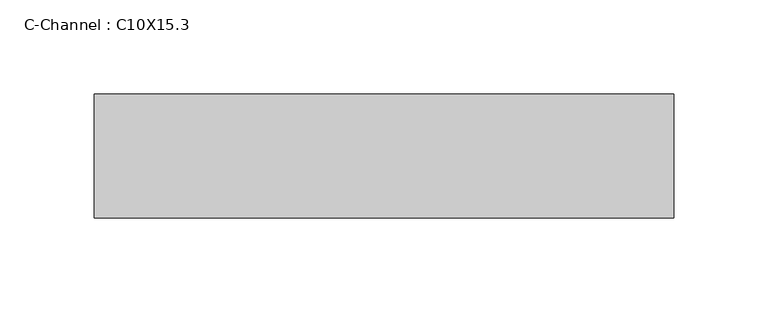
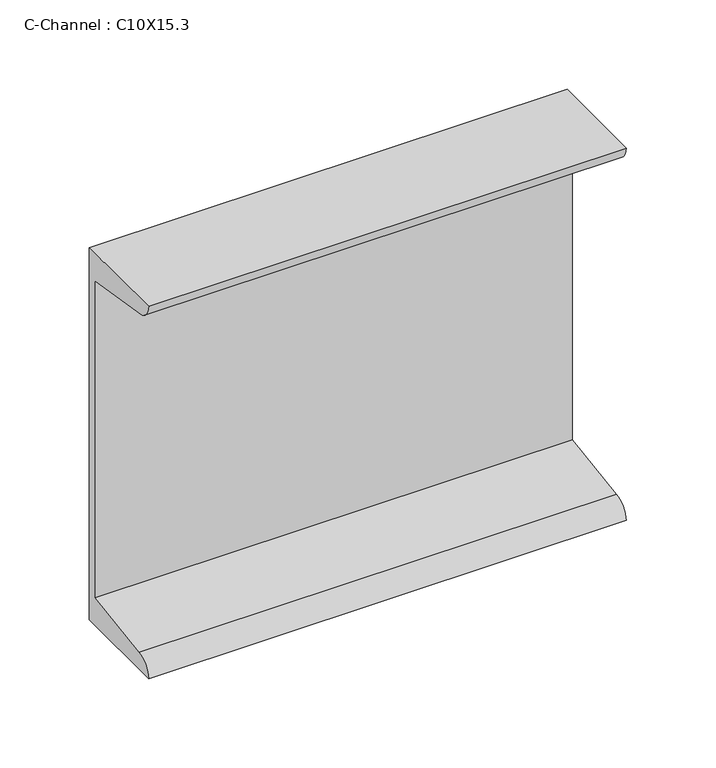
"""IFC4 building model written with IfcOpenShell, lengths in millimetres: beam geometry, C-Channel : C10X15.3."""

from ifc_helpers import new_model, si_unit, point, frame, frame_2d, origin, place, context, project, spatial, polyline, circle_curve, trimmed, segment, composite_curve, outline, extrude, source, transform, mapped, element, save


def c_channel_c10x15_3_af99d691(model_context):
    return source(origin(), model_context, "Body", "SweptSolid", [
        extrude(outline(composite_curve([segment(polyline([(16.1036, 127.0), (16.1036, -127.0), (-49.9364, -127.0)]), True, "CONTINUOUS"), segment(trimmed(circle_curve(frame_2d((-38.862, -127.0)), 11.0744), [point((-49.9364, -127.0))], [point((-38.862, -115.9256))], False, "CARTESIAN"), True, "CONTINUOUS"), segment(polyline([(-38.862, -115.9256), (10.0076, -108.1854158), (10.0076, 108.1854158), (-38.862, 115.9256)]), True, "CONTINUOUS"), segment(trimmed(circle_curve(frame_2d((-38.862, 127.0)), 11.0744), [point((-38.862, 115.9256))], [point((-49.9364, 127.0))], False, "CARTESIAN"), True, "CONTINUOUS"), segment(polyline([(-49.9364, 127.0), (16.1036, 127.0)]), True, "CONTINUOUS")], self_intersect=False)), frame((-155.829, 0.0, 0.0), z_axis=(1.0, 0.0, 0.0), x_axis=(0.0, 1.0, 0.0)), (0.0, 0.0, 1.0), 308.229),
    ])


if __name__ == "__main__":
    model = new_model("IFC4")
    model_context = context("Model", 3, world=origin())
    ifc_project = project(units=[si_unit("LENGTHUNIT", "METRE", prefix="MILLI")], contexts=[model_context])
    site = spatial("IfcSite", under=ifc_project)
    building = spatial("IfcBuilding", under=site)
    placement = place(None, origin())
    c_channel_c10x15_3_shape = c_channel_c10x15_3_af99d691(model_context)
    element("IfcBeam", 1, ObjectType="C-Channel : C10X15.3", at=placement, inside=building, context=model_context, shape_type="MappedRepresentation", body=[
        mapped(c_channel_c10x15_3_shape, transform((0.0, 0.0, 0.0), x_axis=(1.0, 0.0, 0.0), y_axis=(0.0, 1.0, 0.0), z_axis=(0.0, 0.0, 1.0))),
    ])
    save(model, "model.ifc")

# Revit data of these elements
# Type "C-Channel : C10X15.3"
#   Assembly Code = "B10"
#   W = 15.3
#   Length [instance default] = 5' - 0"
#   bf = 0' - 2.6"
#   d = 0' - 10"
#   tf = 0' - 0.436"
#   tw = 0' - 0.24"
#   x = 0' - 0.634"
#   A = 0.0311111 SF
#   Structural Material [instance default] = Steel ASTM A36
# Element 1 (IfcBeam, "C-Channel : C10X15.3")
#   Structural Material = Steel ASTM A992
#   Materials on its faces: "Steel ASTM A992"
# Materials
#   "Steel ASTM A36": class "Metal", colour RGB 199 199 199, transparency 0, Description = "Structural steel, ASTM A36 Grade B, mill finish", Cost = 0
#   "Steel ASTM A992": class "Metal", colour RGB 199 199 199, transparency 0, Description = "Structural steel 50ksi", Cost = 0
